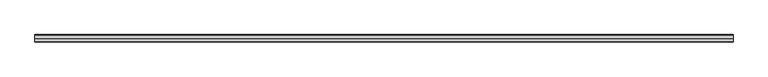
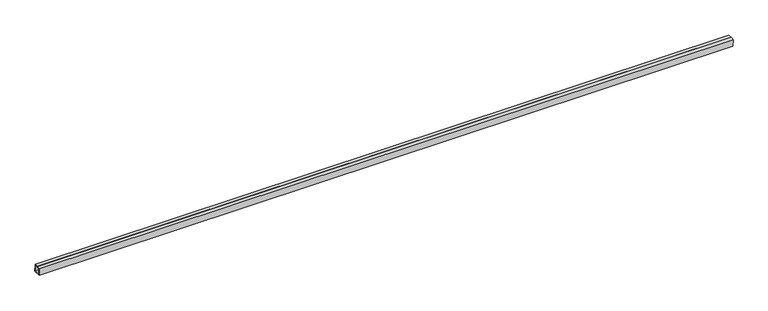
"""IFC4 building model written with IfcOpenShell, lengths in millimetres: proxy geometry, Inner panel:Inner panel:1:Inner panel:1 : Inner panel:Inner panel:300324:2:Inner panel:1:Inner panel:1 : Inner panel:Inner panel:300324:2 : Inner panel:Inner panel:1:Inner panel:1 : Inner panel:Inner panel:300324:300043:52 : Inner panel:Inner panel:1:Inner panel:1 : Inner panel:Inner panel:300324:2:Inner panel:1:Inner panel:1 : Inner panel:Inner panel:300324:2 : Inner panel:Inner panel:1:Inner panel:1 : Inner panel:Inner panel:300324:300043:308120."""

from ifc_helpers import new_model, si_unit, frame, origin, place, context, project, spatial, polyline, outline, extrude, source, transform, mapped, element, save


def generic_models_d6f32502(model_context):
    return source(origin(), model_context, "Body", "SweptSolid", [
        extrude(outline(polyline([(-577258.3887241, 4022.4942957), (-577240.148301, 4023.2543133), (-577238.5621772, 3985.1873432), (-577276.6291473, 3983.6012194), (-577278.215271, 4021.6681895), (-577259.9748479, 4022.4282072), (-577259.8757151, 4020.0490215), (-577275.7369527, 4019.3881366), (-577274.3490944, 3986.0795378), (-577241.0404956, 3987.4673961), (-577242.4283539, 4020.7759949), (-577258.2895914, 4020.11511), (-577258.3887241, 4022.4942957)])), frame((664223.0867238, 0.0, 0.0), z_axis=(1.0, 0.0, 0.0), x_axis=(0.0, 1.0, 0.0)), (0.0, 0.0, 1.0), 3657.6),
    ])


if __name__ == "__main__":
    model = new_model("IFC4")
    model_context = context("Model", 3, world=origin())
    ifc_project = project(units=[si_unit("LENGTHUNIT", "METRE", prefix="MILLI")], contexts=[model_context])
    site = spatial("IfcSite", under=ifc_project)
    building = spatial("IfcBuilding", under=site)
    placement = place(None, origin())
    generic_models_shape = generic_models_d6f32502(model_context)
    element("IfcBuildingElementProxy", 1, Name="Inner panel:Inner panel:1:Inner panel:1 : Inner panel:Inner panel:300324:2:Inner panel:1:Inner panel:1 : Inner panel:Inner panel:300324:2 : Inner panel:Inner panel:1:Inner panel:1 : Inner panel:Inner panel:300324:300043:52 : Inner panel:Inner panel:1:Inner panel:1 : Inner panel:Inner panel:300324:2:Inner panel:1:Inner panel:1 : Inner panel:Inner panel:300324:2 : Inner panel:Inner panel:1:Inner panel:1 : Inner panel:Inner panel:300324:300043:308120", ObjectType="Inner panel:Inner panel:1:Inner panel:1 : Inner panel:Inner panel:300324:2:Inner panel:1:Inner panel:1 : Inner panel:Inner panel:300324:2 : Inner panel:Inner panel:1:Inner panel:1 : Inner panel:Inner panel:300324:300043:52 : Inner panel:Inner panel:1:Inner panel:1 : Inner panel:Inner panel:300324:2:Inner panel:1:Inner panel:1 : Inner panel:Inner panel:300324:2 : Inner panel:Inner panel:1:Inner panel:1 : Inner panel:Inner panel:300324:300043:308120", at=placement, inside=building, context=model_context, shape_type="MappedRepresentation", body=[
        mapped(generic_models_shape, transform((0.0, 0.0, 0.0), x_axis=(1.0, 0.0, 0.0), y_axis=(0.0, 1.0, 0.0), z_axis=(0.0, 0.0, 1.0))),
    ])
    save(model, "model.ifc")

# Revit data of these elements
# Type "Inner panel:Inner panel:1:Inner panel:1 : Inner panel:Inner panel:300324:2:Inner panel:1:Inner panel:1 : Inner panel:Inner panel:300324:2 : Inner panel:Inner panel:1:Inner panel:1 : Inner panel:Inner panel:300324:300043:52 : Inner panel:Inner panel:1:Inner panel:1 : Inner panel:Inner panel:300324:2:Inner panel:1:Inner panel:1 : Inner panel:Inner panel:300324:2 : Inner panel:Inner panel:1:Inner panel:1 : Inner panel:Inner panel:300324:300043:308120"
#   NameOverride = "Inner panel:Inner panel:1:Inner panel:1 : Inner panel:Inner panel:300324:2:Inner panel:1:Inner panel:1 : Inner panel:Inner panel:300324:2 : Inner panel:Inner panel:1:Inner panel:1 : Inner panel:Inner panel:300324:300043:308120"
#   ObjectTypeOverride = "Inner panel:1:Inner panel:1 : Inner panel:Inner panel:300324:2 : Inner panel:Inner panel:1:Inner panel:1 : Inner panel:Inner panel:300324:300043"
#   Reference = "Inner panel"
#   Tag = "308120"
# Element 1 (IfcBuildingElementProxy, "Inner panel:Inner panel:1:Inner panel:1 : Inner panel:Inner panel:300324:2:Inner panel:1:Inner panel:1 : Inner panel:Inner panel:300324:2 : Inner panel:Inner panel:1:Inner panel:1 : Inner panel:Inner panel:300324:300043:52 : Inner panel:Inner panel:1:Inner panel:1 : Inner panel:Inner panel:300324:2:Inner panel:1:Inner panel:1 : Inner panel:Inner panel:300324:2 : Inner panel:Inner panel:1:Inner panel:1 : Inner panel:Inner panel:300324:300043:308120")
#   Materials on its faces: "1 1/2\" X 1 1/2\" SPLIT-SEAM SQUARE TUBING (~24\" CANTILEVER FROM C.L. OF GLULAM)"
# Materials
#   "1 1/2\" X 1 1/2\" SPLIT-SEAM SQUARE TUBING (~24\" CANTILEVER FROM C.L. OF GLULAM)": class "Unassigned", colour RGB 202 201 200, transparency 0, Cost = 0
